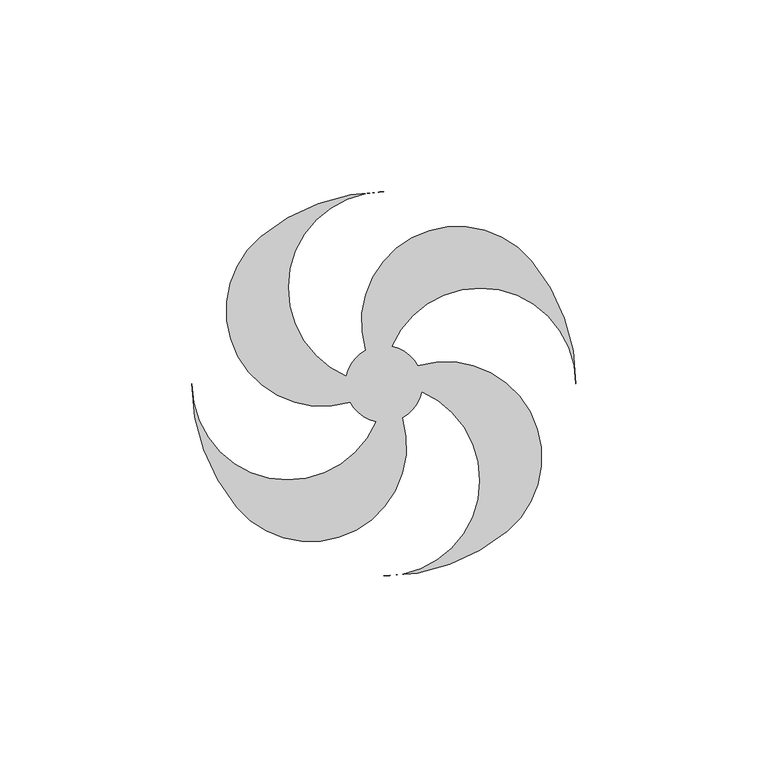
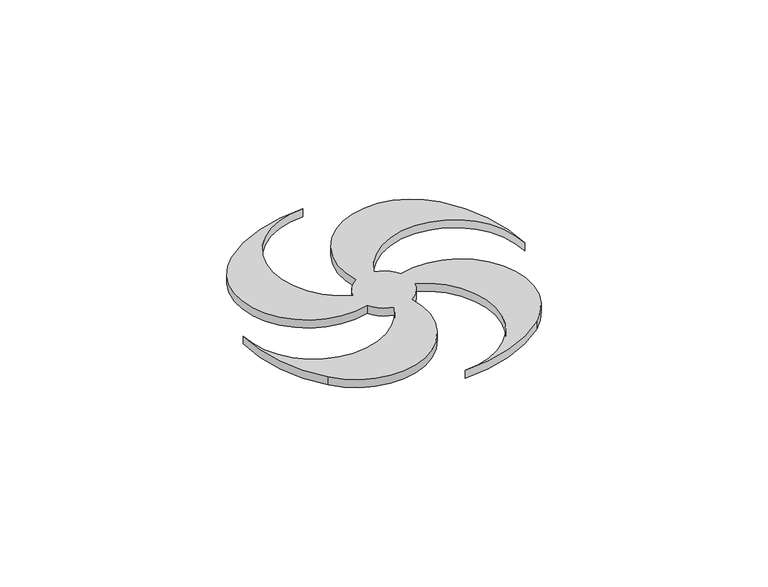
"""IFC4 building model written with IfcOpenShell, lengths in millimetres: proxy geometry, TSP AC Point 24,000-30,000 BTU : TSP AC Point 24,000-30,000 BTU."""

from ifc_helpers import new_model, si_unit, point, frame_2d, origin, origin_with_axes, place, context, project, spatial, circle_curve, trimmed, segment, composite_curve, outline, extrude, source, transform, mapped, element, save


def electrical_fixtures_5faf2b63(model_context):
    return source(origin(), model_context, "Body", "SweptSolid", [
        extrude(outline(composite_curve([segment(trimmed(circle_curve(frame_2d((-50.0, 0.0)), 50.0), [point((-88.3022222, -32.1393805))], [point((-100.0, 0.0))], False, "CARTESIAN"), True, "CONTINUOUS"), segment(trimmed(circle_curve(frame_2d((-75.0, 0.0)), 25.0), [point((-100.0, 0.0))], [point((-52.0, -9.797959))], True, "CARTESIAN"), True, "CONTINUOUS"), segment(trimmed(circle_curve(frame_2d((-50.0, 0.0)), 10.0), [point((-52.0, -9.797959))], [point((-58.7912472, -4.7659177))], False, "CARTESIAN"), True, "CONTINUOUS"), segment(trimmed(circle_curve(frame_2d((-66.0696902, 19.1511111)), 25.0), [point((-58.7912472, -4.7659177))], [point((-82.1393805, 38.3022222))], False, "CARTESIAN"), True, "CONTINUOUS"), segment(trimmed(circle_curve(frame_2d((-50.0, 0.0)), 50.0), [point((-82.1393805, 38.3022222))], [point((-50.0, 50.0))], False, "CARTESIAN"), True, "CONTINUOUS"), segment(trimmed(circle_curve(frame_2d((-50.0, 25.0)), 25.0), [point((-50.0, 50.0))], [point((-59.797959, 2.0))], True, "CARTESIAN"), True, "CONTINUOUS"), segment(trimmed(circle_curve(frame_2d((-50.0, 0.0)), 10.0), [point((-59.797959, 2.0))], [point((-54.7659177, 8.7912472))], False, "CARTESIAN"), True, "CONTINUOUS"), segment(trimmed(circle_curve(frame_2d((-30.8488889, 16.0696902)), 25.0), [point((-54.7659177, 8.7912472))], [point((-11.6977778, 32.1393805))], False, "CARTESIAN"), True, "CONTINUOUS"), segment(trimmed(circle_curve(frame_2d((-50.0, 0.0)), 50.0), [point((-11.6977778, 32.1393805))], [point((0.0, 0.0))], False, "CARTESIAN"), True, "CONTINUOUS"), segment(trimmed(circle_curve(frame_2d((-25.0, 0.0)), 25.0), [point((0.0, 0.0))], [point((-48.0, 9.797959))], True, "CARTESIAN"), True, "CONTINUOUS"), segment(trimmed(circle_curve(frame_2d((-50.0, 0.0)), 10.0), [point((-48.0, 9.797959))], [point((-41.2087528, 4.7659177))], False, "CARTESIAN"), True, "CONTINUOUS"), segment(trimmed(circle_curve(frame_2d((-33.9303098, -19.1511111)), 25.0), [point((-41.2087528, 4.7659177))], [point((-17.8606195, -38.3022222))], False, "CARTESIAN"), True, "CONTINUOUS"), segment(trimmed(circle_curve(frame_2d((-50.0, 0.0)), 50.0), [point((-17.8606195, -38.3022222))], [point((-50.0, -50.0))], False, "CARTESIAN"), True, "CONTINUOUS"), segment(trimmed(circle_curve(frame_2d((-50.0, -25.0)), 25.0), [point((-50.0, -50.0))], [point((-40.202041, -2.0))], True, "CARTESIAN"), True, "CONTINUOUS"), segment(trimmed(circle_curve(frame_2d((-50.0, 0.0)), 10.0), [point((-40.202041, -2.0))], [point((-45.2340823, -8.7912472))], False, "CARTESIAN"), True, "CONTINUOUS"), segment(trimmed(circle_curve(frame_2d((-69.1511111, -16.0696902)), 25.0), [point((-45.2340823, -8.7912472))], [point((-88.3022222, -32.1393805))], False, "CARTESIAN"), True, "CONTINUOUS")], self_intersect=False)), origin_with_axes(), (0.0, 0.0, 1.0), 3.0),
    ])


if __name__ == "__main__":
    model = new_model("IFC4")
    model_context = context("Model", 3, world=origin())
    ifc_project = project(units=[si_unit("LENGTHUNIT", "METRE", prefix="MILLI")], contexts=[model_context])
    site = spatial("IfcSite", under=ifc_project)
    building = spatial("IfcBuilding", under=site)
    placement = place(None, origin())
    electrical_fixtures_shape = electrical_fixtures_5faf2b63(model_context)
    element("IfcBuildingElementProxy", 1, Name="TSP AC Point 24,000-30,000 BTU : TSP AC Point 24,000-30,000 BTU", ObjectType="TSP AC Point 24,000-30,000 BTU : TSP AC Point 24,000-30,000 BTU", at=placement, inside=building, context=model_context, shape_type="MappedRepresentation", body=[
        mapped(electrical_fixtures_shape, transform((0.0, 0.0, 0.0), x_axis=(1.0, 0.0, 0.0), y_axis=(0.0, 1.0, 0.0), z_axis=(0.0, 0.0, 1.0))),
    ])
    save(model, "model.ifc")

# Revit data of these elements
# Type "TSP AC Point 24,000-30,000 BTU : TSP AC Point 24,000-30,000 BTU"
#   Model = "TSP_ELECACP2430"
#   Default Elevation = 0
# Element 1 (IfcBuildingElementProxy, "TSP AC Point 24,000-30,000 BTU : TSP AC Point 24,000-30,000 BTU")
#   Materials on its faces: "Plastic, Opaque Black"
# Materials
#   "Plastic, Opaque Black": class "Plastic", colour RGB 0 0 0, transparency 0.7, Description = "Plastic, generic, opaque black", Cost = 0
